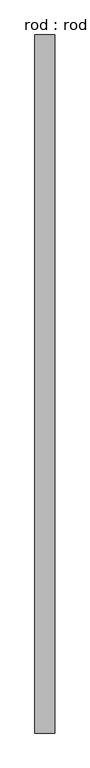
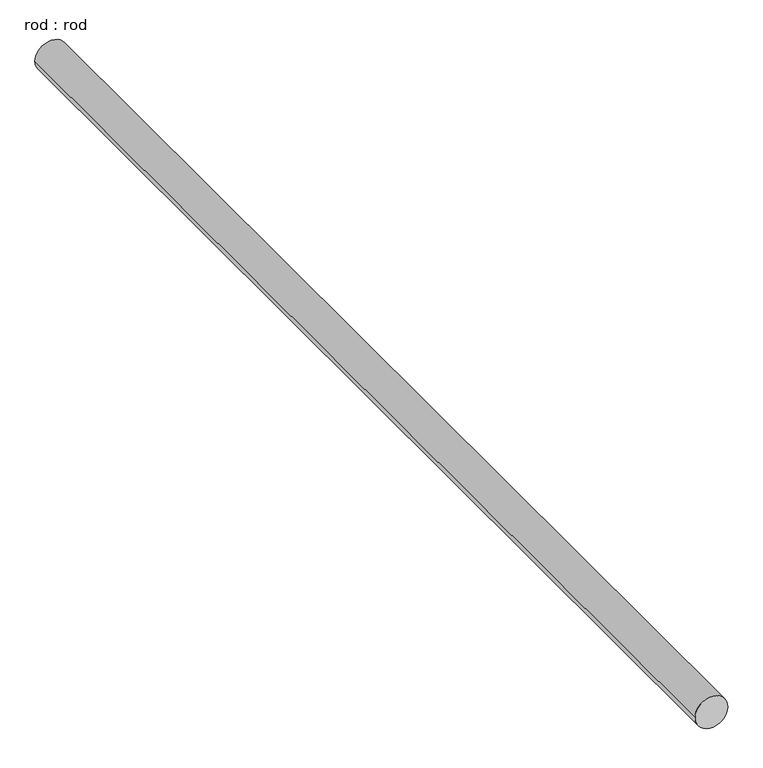
"""IFC4 building model written with IfcOpenShell, lengths in millimetres: proxy geometry, rod : rod."""

from ifc_helpers import new_model, si_unit, point, frame, frame_2d, origin, place, context, project, spatial, circle_curve, trimmed, segment, composite_curve, outline, extrude, source, transform, mapped, element, save


def rod_rod_0d68e6c6(model_context):
    return source(origin(), model_context, "Body", "SweptSolid", [
        extrude(outline(composite_curve([segment(trimmed(circle_curve(frame_2d((0.0108462, 0.0)), 200.0), [point((0.0108462, 200.0))], [point((0.0108462, -200.0))], False, "CARTESIAN"), True, "CONTINUOUS"), segment(trimmed(circle_curve(frame_2d((0.0108462, 0.0)), 200.0), [point((0.0108462, -200.0))], [point((0.0108462, 200.0))], False, "CARTESIAN"), True, "CONTINUOUS")], self_intersect=False)), frame((0.0, -2882.9172567, 0.0), z_axis=(0.0, 1.0, 0.0), x_axis=(0.0, 0.0, 1.0)), (0.0, 0.0, 1.0), 13951.291744),
    ])


if __name__ == "__main__":
    model = new_model("IFC4")
    model_context = context("Model", 3, world=origin())
    ifc_project = project(units=[si_unit("LENGTHUNIT", "METRE", prefix="MILLI")], contexts=[model_context])
    site = spatial("IfcSite", under=ifc_project)
    building = spatial("IfcBuilding", under=site)
    placement = place(None, origin())
    rod_rod_shape = rod_rod_0d68e6c6(model_context)
    element("IfcBuildingElementProxy", 1, Name="rod : rod", ObjectType="rod : rod", at=placement, inside=building, context=model_context, shape_type="MappedRepresentation", body=[
        mapped(rod_rod_shape, transform((0.0, 0.0, 0.0), x_axis=(1.0, 0.0, 0.0), y_axis=(0.0, 1.0, 0.0), z_axis=(0.0, 0.0, 1.0))),
    ])
    save(model, "model.ifc")

# Revit data of these elements
# Type "rod : rod"
#   Default Elevation = 0
